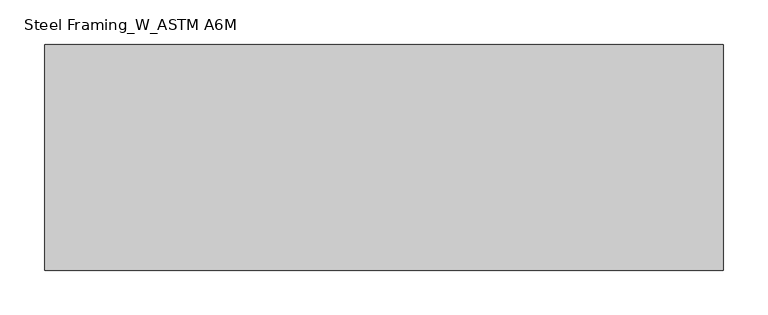
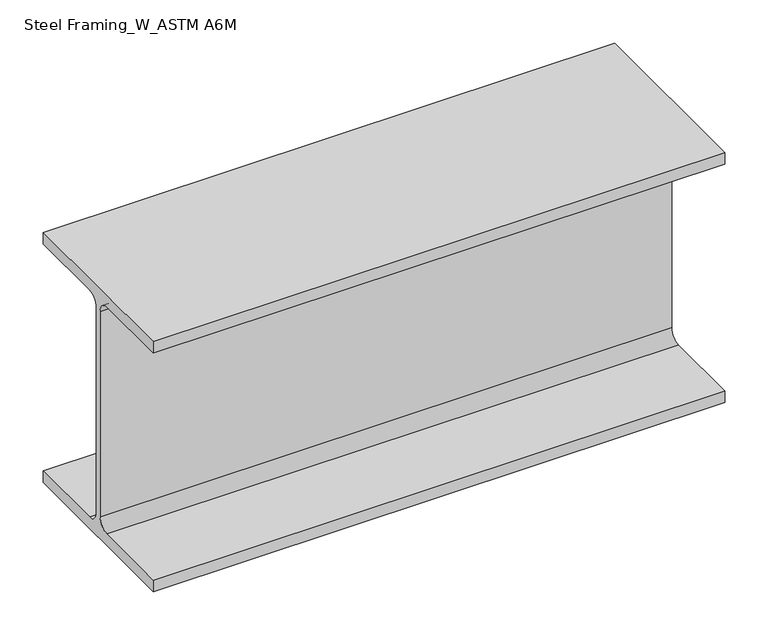
"""IFC4 building model written with IfcOpenShell, lengths in millimetres: beam geometry, Steel Framing_W_ASTM A6M : H_SB_AR_S02_W360x91_B3."""

from ifc_helpers import new_model, si_unit, point, frame, frame_2d, origin, place, context, project, spatial, polyline, circle_curve, trimmed, segment, composite_curve, outline, extrude, source, transform, mapped, element, save


def steel_framing_w_astm_a6m_e4d07942(model_context):
    return source(origin(), model_context, "Body", "SweptSolid", [
        extrude(outline(composite_curve([segment(polyline([(127.0, -160.1), (127.0, -176.5), (-127.0, -176.5), (-127.0, -160.1), (-19.865, -160.1)]), True, "CONTINUOUS"), segment(trimmed(circle_curve(frame_2d((-19.865, -145.0)), 15.1), [point((-19.865, -160.1))], [point((-4.765, -145.0))], True, "CARTESIAN"), True, "CONTINUOUS"), segment(polyline([(-4.765, -145.0), (-4.765, 145.0)]), True, "CONTINUOUS"), segment(trimmed(circle_curve(frame_2d((-19.865, 145.0)), 15.1), [point((-4.765, 145.0))], [point((-19.865, 160.1))], True, "CARTESIAN"), True, "CONTINUOUS"), segment(polyline([(-19.865, 160.1), (-127.0, 160.1), (-127.0, 176.5), (127.0, 176.5), (127.0, 160.1), (19.865, 160.1)]), True, "CONTINUOUS"), segment(trimmed(circle_curve(frame_2d((19.865, 145.0)), 15.1), [point((19.865, 160.1))], [point((4.765, 145.0))], True, "CARTESIAN"), True, "CONTINUOUS"), segment(polyline([(4.765, 145.0), (4.765, -145.0)]), True, "CONTINUOUS"), segment(trimmed(circle_curve(frame_2d((19.865, -145.0)), 15.1), [point((4.765, -145.0))], [point((19.865, -160.1))], True, "CARTESIAN"), True, "CONTINUOUS"), segment(polyline([(19.865, -160.1), (127.0, -160.1)]), True, "CONTINUOUS")], self_intersect=False)), frame((-360.3, 0.0, 0.0), z_axis=(1.0, 0.0, 0.0), x_axis=(0.0, 1.0, 0.0)), (0.0, 0.0, 1.0), 762.1),
    ])


if __name__ == "__main__":
    model = new_model("IFC4")
    model_context = context("Model", 3, world=origin())
    ifc_project = project(units=[si_unit("LENGTHUNIT", "METRE", prefix="MILLI")], contexts=[model_context])
    site = spatial("IfcSite", under=ifc_project)
    building = spatial("IfcBuilding", under=site)
    placement = place(None, origin())
    steel_framing_w_astm_a6m_shape = steel_framing_w_astm_a6m_e4d07942(model_context)
    element("IfcBeam", 1, ObjectType="Steel Framing_W_ASTM A6M : H_SB_AR_S02_W360x91_B3", at=placement, inside=building, context=model_context, shape_type="MappedRepresentation", body=[
        mapped(steel_framing_w_astm_a6m_shape, transform((0.0, 0.0, 0.0), x_axis=(1.0, 0.0, 0.0), y_axis=(0.0, 1.0, 0.0), z_axis=(0.0, 0.0, 1.0))),
    ])
    save(model, "model.ifc")

# Revit data of these elements
# Type "Steel Framing_W_ASTM A6M : H_SB_AR_S02_W360x91_B3"
#   Type Mark = "B3"
#   Section Name Key = "W14x61"
#   Width = 25.4 cm
#   Web Thickness = 0.953 cm
#   Web Fillet = 1.51 cm
#   Warping Constant = 1260000.0 cm⁶
#   Torsional Moment of Inertia = 91.20 cm⁴
#   Section Area = 115.0 cm²
#   Plastic Modulus weak axis = 537.0 cm³
#   Plastic Modulus strong axis = 1670.0 cm³
#   Perimeter = 1.68 m²/m
#   Nominal Weight = 91.00 kgf/m
#   Moment of Inertia weak axis = 4450.00 cm⁴
#   Moment of Inertia strong axis = 26600.00 cm⁴
#   Height = 35.3 cm
#   Flange Thickness = 1.64 cm
#   Elastic Modulus weak axis = 352.0 cm³
#   Elastic Modulus strong axis = 1510.0 cm³
#   Centroid Vertical = 17.65 cm
#   Centroid Horizontal = 12.7 cm
#   Length [instance default] = 1500 mm
#   Structural Material [instance default] = Steel, 45-345
#   Bolt Spacing = 0
#   Assembly Code = ""
# Element 1 (IfcBeam, "Steel Framing_W_ASTM A6M : H_SB_AR_S02_W360x91_B3")
#   Materials on its faces: "Steel, 45-345"
# Materials
#   "Steel, 45-345": class "Metal", colour RGB 189 187 185, transparency 0, Description = "Steel 345 MPa", Cost = 0
